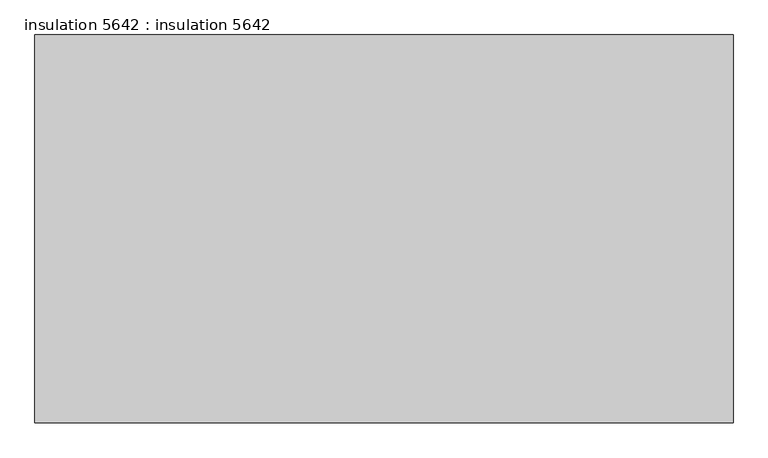
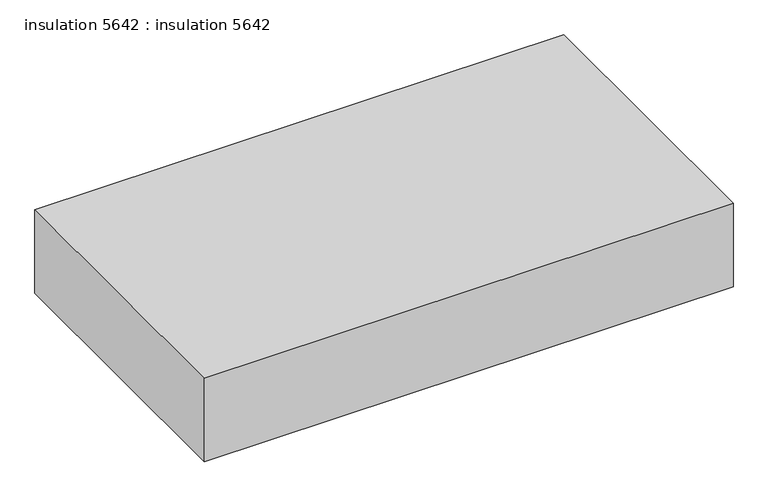
"""IFC4 building model written with IfcOpenShell, lengths in millimetres: proxy geometry, insulation 5642 : insulation 5642."""

from ifc_helpers import new_model, si_unit, frame, origin, place, context, project, spatial, polyline, outline, extrude, source, transform, mapped, element, save


def insulation_5642_insulation_5642_4b85f5e8(model_context):
    return source(origin(), model_context, "Body", "SweptSolid", [
        extrude(outline(polyline([(14211.8178845, -4386.7175368), (14211.8178845, -5402.7175368), (12383.0178845, -5402.7175368), (12383.0178845, -4386.7175368), (14211.8178845, -4386.7175368)])), frame((0.0, 0.0, 39757.096), z_axis=(0.0, 0.0, 1.0), x_axis=(1.0, 0.0, 0.0)), (0.0, 0.0, 1.0), 304.8),
    ])


if __name__ == "__main__":
    model = new_model("IFC4")
    model_context = context("Model", 3, world=origin())
    ifc_project = project(units=[si_unit("LENGTHUNIT", "METRE", prefix="MILLI")], contexts=[model_context])
    site = spatial("IfcSite", under=ifc_project)
    building = spatial("IfcBuilding", under=site)
    placement = place(None, origin())
    insulation_5642_insulation_5642_shape = insulation_5642_insulation_5642_4b85f5e8(model_context)
    element("IfcBuildingElementProxy", 1, Name="insulation 5642 : insulation 5642", ObjectType="insulation 5642 : insulation 5642", at=placement, inside=building, context=model_context, shape_type="MappedRepresentation", body=[
        mapped(insulation_5642_insulation_5642_shape, transform((0.0, 0.0, 0.0), x_axis=(1.0, 0.0, 0.0), y_axis=(0.0, 1.0, 0.0), z_axis=(0.0, 0.0, 1.0))),
    ])
    save(model, "model.ifc")

# Revit data of these elements
# Type "insulation 5642 : insulation 5642"
#   NameOverride = "insulation"
# Element 1 (IfcBuildingElementProxy, "insulation 5642 : insulation 5642")
#   Materials on its faces: "BATT INSULATION (U-FACTOR = 0.065 MIN.) OVER CLASS II VAPOR RETARDER (TOWARDS INTERIOR)"
# Materials
#   "BATT INSULATION (U-FACTOR = 0.065 MIN.) OVER CLASS II VAPOR RETARDER (TOWARDS INTERIOR)": class "Unassigned", colour RGB 246 242 160, transparency 0, Cost = 0
